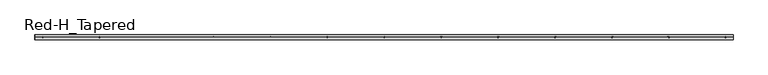
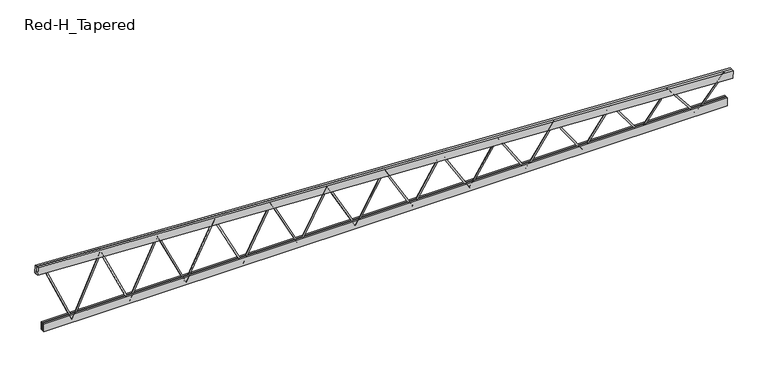
"""IFC4 building model written with IfcOpenShell, lengths in millimetres: beam geometry, Construction_Frames_RedBuilt_Openweb_Red-H_Tapered : Red-H_Tapered."""

from ifc_helpers import new_model, si_unit, point, frame, origin, origin_2d, place, context, project, spatial, polyline, circle_curve, trimmed, segment, composite_curve, outline, extrude, source, transform, mapped, element, save


def red_h_tapered_021202b6(model_context):
    return source(origin(), model_context, "Body", "SweptSolid", [
        extrude(outline(composite_curve([segment(trimmed(circle_curve(origin_2d(), 12.7), [point((0.0, 12.7))], [point((0.0, -12.7))], False, "CARTESIAN"), True, "CONTINUOUS"), segment(trimmed(circle_curve(origin_2d(), 12.7), [point((0.0, -12.7))], [point((0.0, 12.7))], False, "CARTESIAN"), True, "CONTINUOUS")], self_intersect=False)), frame((5452.665625, 0.0, -367.0101562), z_axis=(0.646986574748216, 0.0, 0.7625013915368097), x_axis=(0.0, -1.0, 0.0)), (0.0, 0.0, 1.0), 766.1625362),
        extrude(outline(composite_curve([segment(trimmed(circle_curve(origin_2d(), 12.7), [point((0.0, -12.7000001))], [point((0.0, 12.7))], False, "CARTESIAN"), True, "CONTINUOUS"), segment(trimmed(circle_curve(origin_2d(), 12.7), [point((0.0, 12.7))], [point((0.0, -12.7000001))], False, "CARTESIAN"), True, "CONTINUOUS")], self_intersect=False)), frame((5452.665625, 0.0, -367.0101562), z_axis=(-0.618861229601663, 0.0, 0.7855003364072596), x_axis=(0.0, -1.0, 0.0)), (0.0, 0.0, 1.0), 800.982274),
        extrude(outline(composite_curve([segment(trimmed(circle_curve(origin_2d(), 12.7), [point((0.0, 12.7000001))], [point((0.0, -12.7))], False, "CARTESIAN"), True, "CONTINUOUS"), segment(trimmed(circle_curve(origin_2d(), 12.7), [point((0.0, -12.7))], [point((0.0, 12.7000001))], False, "CARTESIAN"), True, "CONTINUOUS")], self_intersect=False)), frame((4461.271875, 0.0, -367.0101562), z_axis=(0.6188612296016608, 0.0, 0.7855003364072612), x_axis=(0.0, -1.0, 0.0)), (0.0, 0.0, 1.0), 800.982274),
        extrude(outline(composite_curve([segment(trimmed(circle_curve(origin_2d(), 12.7), [point((0.0, -12.7))], [point((0.0, 12.7))], False, "CARTESIAN"), True, "CONTINUOUS"), segment(trimmed(circle_curve(origin_2d(), 12.7), [point((0.0, 12.7))], [point((0.0, -12.7))], False, "CARTESIAN"), True, "CONTINUOUS")], self_intersect=False)), frame((4461.271875, 0.0, -367.0101562), z_axis=(-0.5923927653210783, 0.0, 0.8056493105534479), x_axis=(0.0, -1.0, 0.0)), (0.0, 0.0, 1.0), 836.7706428),
        extrude(outline(composite_curve([segment(trimmed(circle_curve(origin_2d(), 12.7), [point((0.0, 12.7))], [point((0.0, -12.7))], False, "CARTESIAN"), True, "CONTINUOUS"), segment(trimmed(circle_curve(origin_2d(), 12.7), [point((0.0, -12.7))], [point((0.0, 12.7))], False, "CARTESIAN"), True, "CONTINUOUS")], self_intersect=False)), frame((3469.878125, 0.0, -367.0101562), z_axis=(0.592392765321077, 0.0, 0.8056493105534488), x_axis=(0.0, -1.0, 0.0)), (0.0, 0.0, 1.0), 836.7706428),
        extrude(outline(composite_curve([segment(trimmed(circle_curve(origin_2d(), 12.7), [point((0.0, -12.7))], [point((0.0, 12.6999999))], False, "CARTESIAN"), True, "CONTINUOUS"), segment(trimmed(circle_curve(origin_2d(), 12.7), [point((0.0, 12.6999999))], [point((0.0, -12.7))], False, "CARTESIAN"), True, "CONTINUOUS")], self_intersect=False)), frame((3469.878125, 0.0, -367.0101562), z_axis=(-0.5675429419222507, 0.0, 0.8233437976169109), x_axis=(0.0, -1.0, 0.0)), (0.0, 0.0, 1.0), 873.40858),
        extrude(outline(composite_curve([segment(trimmed(circle_curve(origin_2d(), 12.7), [point((0.0, 12.7))], [point((0.0, -12.6999999))], False, "CARTESIAN"), True, "CONTINUOUS"), segment(trimmed(circle_curve(origin_2d(), 12.7), [point((0.0, -12.6999999))], [point((0.0, 12.7))], False, "CARTESIAN"), True, "CONTINUOUS")], self_intersect=False)), frame((2478.484375, 0.0, -367.0101562), z_axis=(0.5675429419222516, 0.0, 0.8233437976169103), x_axis=(0.0, -1.0, 0.0)), (0.0, 0.0, 1.0), 873.40858),
        extrude(outline(composite_curve([segment(trimmed(circle_curve(origin_2d(), 12.7), [point((0.0, -12.7000001))], [point((0.0, 12.7))], False, "CARTESIAN"), True, "CONTINUOUS"), segment(trimmed(circle_curve(origin_2d(), 12.7), [point((0.0, 12.7))], [point((0.0, -12.7000001))], False, "CARTESIAN"), True, "CONTINUOUS")], self_intersect=False)), frame((2478.484375, 0.0, -367.0101562), z_axis=(-0.5442472293507187, 0.0, 0.8389248794403861), x_axis=(0.0, -1.0, 0.0)), (0.0, 0.0, 1.0), 910.7935664),
        extrude(outline(composite_curve([segment(trimmed(circle_curve(origin_2d(), 12.7), [point((0.0, 12.7000001))], [point((0.0, -12.7))], False, "CARTESIAN"), True, "CONTINUOUS"), segment(trimmed(circle_curve(origin_2d(), 12.7), [point((0.0, -12.7))], [point((0.0, 12.7000001))], False, "CARTESIAN"), True, "CONTINUOUS")], self_intersect=False)), frame((1487.090625, 0.0, -367.0101562), z_axis=(0.5442472293507231, 0.0, 0.8389248794403832), x_axis=(0.0, -1.0, 0.0)), (0.0, 0.0, 1.0), 910.7935664),
        extrude(outline(composite_curve([segment(trimmed(circle_curve(origin_2d(), 12.7), [point((0.0, -12.7000001))], [point((0.0, 12.7))], False, "CARTESIAN"), True, "CONTINUOUS"), segment(trimmed(circle_curve(origin_2d(), 12.7), [point((0.0, 12.7))], [point((0.0, -12.7000001))], False, "CARTESIAN"), True, "CONTINUOUS")], self_intersect=False)), frame((1487.090625, 0.0, -367.0101562), z_axis=(-0.5224255765774791, 0.0, 0.8526848872459794), x_axis=(0.0, -1.0, 0.0)), (0.0, 0.0, 1.0), 948.8373028),
        extrude(outline(composite_curve([segment(trimmed(circle_curve(origin_2d(), 12.7), [point((0.0, 12.7000001))], [point((0.0, -12.7))], False, "CARTESIAN"), True, "CONTINUOUS"), segment(trimmed(circle_curve(origin_2d(), 12.7), [point((0.0, -12.7))], [point((0.0, 12.7000001))], False, "CARTESIAN"), True, "CONTINUOUS")], self_intersect=False)), frame((495.696875, 0.0, -367.0101562), z_axis=(0.5224255765774808, 0.0, 0.8526848872459784), x_axis=(0.0, -1.0, 0.0)), (0.0, 0.0, 1.0), 948.8373028),
        extrude(outline(composite_curve([segment(trimmed(circle_curve(origin_2d(), 12.7), [point((0.0, -12.7))], [point((0.0, 12.7))], False, "CARTESIAN"), True, "CONTINUOUS"), segment(trimmed(circle_curve(origin_2d(), 12.7), [point((0.0, 12.7))], [point((0.0, -12.7))], False, "CARTESIAN"), True, "CONTINUOUS")], self_intersect=False)), frame((495.696875, 0.0, -367.0101562), z_axis=(-0.5019899953354453, 0.0, 0.8648734269146668), x_axis=(0.0, -1.0, 0.0)), (0.0, 0.0, 1.0), 987.4636539),
        extrude(outline(composite_curve([segment(trimmed(circle_curve(origin_2d(), 12.7), [point((0.0, 12.7))], [point((0.0, -12.7))], False, "CARTESIAN"), True, "CONTINUOUS"), segment(trimmed(circle_curve(origin_2d(), 12.7), [point((0.0, -12.7))], [point((0.0, 12.7))], False, "CARTESIAN"), True, "CONTINUOUS")], self_intersect=False)), frame((-495.696875, 0.0, -367.0101562), z_axis=(0.5019899953354093, 0.0, 0.8648734269146878), x_axis=(0.0, -1.0, 0.0)), (0.0, 0.0, 1.0), 987.4636539),
        extrude(outline(composite_curve([segment(trimmed(circle_curve(origin_2d(), 12.7), [point((0.0, -12.7))], [point((0.0, 12.6999999))], False, "CARTESIAN"), True, "CONTINUOUS"), segment(trimmed(circle_curve(origin_2d(), 12.7), [point((0.0, 12.6999999))], [point((0.0, -12.7))], False, "CARTESIAN"), True, "CONTINUOUS")], self_intersect=False)), frame((-495.696875, 0.0, -367.0101562), z_axis=(-0.48284975973910615, 0.0, 0.8757032085814734), x_axis=(0.0, -1.0, 0.0)), (0.0, 0.0, 1.0), 1026.6068586),
        extrude(outline(composite_curve([segment(trimmed(circle_curve(origin_2d(), 12.7), [point((0.0, 12.7))], [point((0.0, -12.6999999))], False, "CARTESIAN"), True, "CONTINUOUS"), segment(trimmed(circle_curve(origin_2d(), 12.7), [point((0.0, -12.6999999))], [point((0.0, 12.7))], False, "CARTESIAN"), True, "CONTINUOUS")], self_intersect=False)), frame((-1487.090625, 0.0, -367.0101562), z_axis=(0.48284975973910677, 0.0, 0.875703208581473), x_axis=(0.0, -1.0, 0.0)), (0.0, 0.0, 1.0), 1026.6068586),
        extrude(outline(composite_curve([segment(trimmed(circle_curve(origin_2d(), 12.7), [point((0.0, -12.7))], [point((0.0, 12.7))], False, "CARTESIAN"), True, "CONTINUOUS"), segment(trimmed(circle_curve(origin_2d(), 12.7), [point((0.0, 12.7))], [point((0.0, -12.7))], False, "CARTESIAN"), True, "CONTINUOUS")], self_intersect=False)), frame((-1487.090625, 0.0, -367.0101562), z_axis=(-0.4649148648371085, 0.0, 0.885355391045592), x_axis=(0.0, -1.0, 0.0)), (0.0, 0.0, 1.0), 1066.2099935),
        extrude(outline(composite_curve([segment(trimmed(circle_curve(origin_2d(), 12.7), [point((0.0, -12.7))], [point((0.0, 12.7))], False, "CARTESIAN"), True, "CONTINUOUS"), segment(trimmed(circle_curve(origin_2d(), 12.7), [point((0.0, 12.7))], [point((0.0, -12.7))], False, "CARTESIAN"), True, "CONTINUOUS")], self_intersect=False)), frame((-2478.484375, 0.0, -367.0101562), z_axis=(0.4649148648371126, 0.0, 0.8853553910455899), x_axis=(0.0, -1.0, 0.0)), (0.0, 0.0, 1.0), 1066.2099935),
        extrude(outline(composite_curve([segment(trimmed(circle_curve(origin_2d(), 12.7), [point((0.0, 12.7))], [point((0.0, -12.7))], False, "CARTESIAN"), True, "CONTINUOUS"), segment(trimmed(circle_curve(origin_2d(), 12.7), [point((0.0, -12.7))], [point((0.0, 12.7))], False, "CARTESIAN"), True, "CONTINUOUS")], self_intersect=False)), frame((-2478.484375, 0.0, -367.0101562), z_axis=(-0.44809823878717214, 0.0, 0.8939843222315671), x_axis=(0.0, -1.0, 0.0)), (0.0, 0.0, 1.0), 1106.2236628),
        extrude(outline(composite_curve([segment(trimmed(circle_curve(origin_2d(), 12.7), [point((0.0, -12.7))], [point((0.0, 12.7))], False, "CARTESIAN"), True, "CONTINUOUS"), segment(trimmed(circle_curve(origin_2d(), 12.7), [point((0.0, 12.7))], [point((0.0, -12.7))], False, "CARTESIAN"), True, "CONTINUOUS")], self_intersect=False)), frame((-3469.878125, 0.0, -367.0101562), z_axis=(0.44809823878717164, 0.0, 0.8939843222315674), x_axis=(0.0, -1.0, 0.0)), (0.0, 0.0, 1.0), 1106.2236628),
        extrude(outline(composite_curve([segment(trimmed(circle_curve(origin_2d(), 12.7), [point((0.0, 12.6999999))], [point((0.0, -12.7))], False, "CARTESIAN"), True, "CONTINUOUS"), segment(trimmed(circle_curve(origin_2d(), 12.7), [point((0.0, -12.7))], [point((0.0, 12.6999999))], False, "CARTESIAN"), True, "CONTINUOUS")], self_intersect=False)), frame((-3469.878125, 0.0, -367.0101562), z_axis=(-0.432317078389782, 0.0, 0.9017216553529827), x_axis=(0.0, -1.0, 0.0)), (0.0, 0.0, 1.0), 1146.6048874),
        extrude(outline(composite_curve([segment(trimmed(circle_curve(origin_2d(), 12.7), [point((0.0, -12.6999999))], [point((0.0, 12.7))], False, "CARTESIAN"), True, "CONTINUOUS"), segment(trimmed(circle_curve(origin_2d(), 12.7), [point((0.0, 12.7))], [point((0.0, -12.6999999))], False, "CARTESIAN"), True, "CONTINUOUS")], self_intersect=False)), frame((-4461.271875, 0.0, -367.0101562), z_axis=(0.4323170783897885, 0.0, 0.9017216553529794), x_axis=(0.0, -1.0, 0.0)), (0.0, 0.0, 1.0), 1146.6048874),
        extrude(outline(composite_curve([segment(trimmed(circle_curve(origin_2d(), 12.7), [point((0.0, 12.7))], [point((0.0, -12.7))], False, "CARTESIAN"), True, "CONTINUOUS"), segment(trimmed(circle_curve(origin_2d(), 12.7), [point((0.0, -12.7))], [point((0.0, 12.7))], False, "CARTESIAN"), True, "CONTINUOUS")], self_intersect=False)), frame((-4461.271875, 0.0, -367.0101562), z_axis=(-0.41749357862727726, 0.0, 0.9086798731153836), x_axis=(0.0, -1.0, 0.0)), (0.0, 0.0, 1.0), 1187.3161657),
        extrude(outline(composite_curve([segment(trimmed(circle_curve(origin_2d(), 12.7), [point((0.0, -12.7))], [point((0.0, 12.7))], False, "CARTESIAN"), True, "CONTINUOUS"), segment(trimmed(circle_curve(origin_2d(), 12.7), [point((0.0, 12.7))], [point((0.0, -12.7))], False, "CARTESIAN"), True, "CONTINUOUS")], self_intersect=False)), frame((-5452.665625, 0.0, -367.0101562), z_axis=(0.41749357862727704, 0.0, 0.9086798731153837), x_axis=(0.0, -1.0, 0.0)), (0.0, 0.0, 1.0), 1187.3161657),
        extrude(outline(composite_curve([segment(trimmed(circle_curve(origin_2d(), 12.7), [point((0.0, 12.6999999))], [point((0.0, -12.7))], False, "CARTESIAN"), True, "CONTINUOUS"), segment(trimmed(circle_curve(origin_2d(), 12.7), [point((0.0, -12.7))], [point((0.0, 12.6999999))], False, "CARTESIAN"), True, "CONTINUOUS")], self_intersect=False)), frame((-5452.665625, 0.0, -367.0101562), z_axis=(-0.4035552511902556, 0.0, 0.9149552771784912), x_axis=(0.0, -1.0, 0.0)), (0.0, 0.0, 1.0), 1228.3246805),
        extrude(outline(polyline([(-5973.7625, -41.275), (-5973.7625, -3.175), (5973.7625, -3.175), (5973.7625, -41.275), (-5973.7625, -41.275)])), frame((0.0, 0.0, -386.0601562), z_axis=(0.0, 0.0, 1.0), x_axis=(1.0, 0.0, 0.0)), (0.0, 0.0, 1.0), 139.7),
        extrude(outline(polyline([(-5973.7625, 3.175), (-5973.7625, 41.275), (5973.7625, 41.275), (5973.7625, 3.175), (-5973.7625, 3.175)])), frame((0.0, 0.0, -386.0601562), z_axis=(0.0, 0.0, 1.0), x_axis=(1.0, 0.0, 0.0)), (0.0, 0.0, 1.0), 139.7),
        extrude(outline(polyline([(0.0, -38.1), (0.0, 0.0), (12166.0071587, 0.0), (12166.0071587, -38.1), (0.0, -38.1)])), frame((-6082.3624235, -3.175, 693.6153259), z_axis=(0.050106825686347715, 0.0, 0.9987438640710831), x_axis=(0.9987438640710831, 0.0, -0.050106825686347715)), (0.0, 0.0, 1.0), 139.7),
        extrude(outline(polyline([(0.0, -38.1), (0.0, 0.0), (12166.0071587, 0.0), (12166.0071587, -38.1), (0.0, -38.1)])), frame((-6082.3624235, 41.275, 693.6153259), z_axis=(0.050106825686347715, 0.0, 0.9987438640710831), x_axis=(0.9987438640710831, 0.0, -0.050106825686347715)), (0.0, 0.0, 1.0), 139.7),
    ])


if __name__ == "__main__":
    model = new_model("IFC4")
    model_context = context("Model", 3, world=origin())
    ifc_project = project(units=[si_unit("LENGTHUNIT", "METRE", prefix="MILLI")], contexts=[model_context])
    site = spatial("IfcSite", under=ifc_project)
    building = spatial("IfcBuilding", under=site)
    placement = place(None, origin())
    red_h_tapered_shape = red_h_tapered_021202b6(model_context)
    element("IfcBeam", 1, ObjectType="Construction_Frames_RedBuilt_Openweb_Red-H_Tapered : Red-H_Tapered", at=placement, inside=building, context=model_context, shape_type="MappedRepresentation", body=[
        mapped(red_h_tapered_shape, transform((0.0, 0.0, 0.0), x_axis=(1.0, 0.0, 0.0), y_axis=(0.0, 1.0, 0.0), z_axis=(0.0, 0.0, 1.0))),
    ])
    save(model, "model.ifc")

# Revit data of these elements
# Project information
#   Project Issue Date = "05/02/2019"
#   Project Status = "Project Status"
#   Client Name = "Owner"
#   Project Address = "SOMERS, WI"
#   Project Name = "OAKFIRE 2.0"
#   Project Number = "Project Number"
# Type "Construction_Frames_RedBuilt_Openweb_Red-H_Tapered : Red-H_Tapered"
#   Youtube clip = ""
#   Weight Net (Kg) = "0"
#   Webs = "Up to 2\" diameter tubular steel"
#   Uniformat II Description = ""
#   Uniformat II Code = ""
#   Uniclass 2015 Name = "Softwood trusses"
#   Uniclass 2015 Code = "Pr_20_85_90_81"
#   Uniclass 2.0 Description = "Structural Framing Systems"
#   Uniclass 2.0 Code = "SS-15-10-75"
#   Uniclass 1.4 Description = "Trusses"
#   Uniclass 1.4 Code = "L3523"
#   UNSPSC Code = "30103606"
#   Technical description = "http://www.redbuilt.com/reference/literature-and-other-resources"
#   Region South America = "None"
#   Region Oceania = "None"
#   Region North America = "US"
#   Region Middle East = "None"
#   Region Europe = "None"
#   Region Asia = "None"
#   Region Antarctica = "None"
#   Region Africa = "None"
#   QR code = "http://bimobject.com/redbuilt/product/redbuilt-0003"
#   Product url = "http://www.redbuilt.com/products/default.aspx?id=2"
#   Product group = "Wood Trusses"
#   Product family = "Construction"
#   Product data url = "https://bimobject.com/redbuilt/product/redbuilt-0003"
#   Product certification = ""
#   Product SKU = "redbuilt-0003"
#   Product Page URL = "http://www.redbuilt.com/commercial-systems/red-m-red-h-open-web-trusses"
#   Product Guid = "2c5793f2-6ffb-4665-b825-cf90c048e711"
#   Product Documentation Link = "http://www.redbuilt.com/documents/OW_Guide_2017_07_LowRes_wLinks.pdf"
#   OmniClass Description = "Wood Trusses"
#   OmniClass Code = "23-13 35 19 13 17"
#   NBS Reference Description = ""
#   NBS Reference Code = ""
#   Material secondary = "Steel"
#   Material main = "Wood"
#   Masterformat 2014 Description = "Metal-Web Wood Joists"
#   Masterformat 2014 Code = "06 17 36"
#   Manufacturer name = "RedBuilt"
#   Manufacturer country = "United States"
#   Installation instructions = "http://www.redbuilt.com/documents/Installation_Sheets_Open-Web.pdf"
#   IFC Classification = ""
#   EAN code = ""
#   Design country = "United States"
#   Product Information = "http://redbuilt.com/products/default.aspx?id=2"
#   Model = "Red-H-Tapered"
#   Manufacturer URL = "http://redbuilt.com/"
#   Manufacturer = "RedBuilt™"
#   Description = "Open Web Truss"
#   Date of publishing = "8/17/2010"
#   Contact us = "http://redbuilt.com/contact/"
#   Chords = "Double 1½\" x 5½\" MSR lumber"
#   COBIe Type Category = ""
#   Brand url = "http://www.redbuilt.com"
#   BIMobject main category code = "construction"
#   BIMobject main category = "Construction"
#   BIMobject category code = "construction-frames-trusses"
#   BIMobject category = "Frames & Trusses"
#   Web Radius = 0' - 0 1/2"
#   Web Layout Offset Start [instance default] = 0' - 5"
#   Web Layout Offset End [instance default] = 0' - 5"
#   Web Diameter = 0' - 1"
#   TotalLength [instance default] = 20' - 0"
#   Span Minimum = 4' - 0"
#   Span Maximum = 70' - 0"
#   Span Limit [instance default] = 20' - 0"
#   Nominal width = 0' - 0"
#   Nominal height = 0' - 0"
#   Inner Depth Top [instance default] = 0' - 2.76372"
#   Depth Start [instance default] = 6' - 0"
#   Top Chord Length [instance default] = 20' - 1.19701"
#   TC Extension Start Aux [instance default] = 0' - 0"
#   TC Extension End Aux [instance default] = 0' - 0"
#   T-B Chord Length Difference L [instance default] = 0' - 4"
#   T-B Chord Length Difference [instance default] = 0' - 4"
#   Height 2 [instance default] = 6' - 0"
#   Depth Minimum at Wall = 2' - 0"
#   Depth Maximum at Wall = 6' - 0"
#   Depth Lower End [instance default] = 2' - 0"
#   Depth Higher End [instance default] = 6' - 0"
#   Depth End [instance default] = 2' - 0"
#   Depth 2 [instance default] = 2' - 0"
#   Chord Width = 0' - 3 1/4"
#   Chord Thickness = 0' - 1 1/2"
#   Chord Depth = 0' - 5 1/2"
#   Offset Start [instance default] = 0' - 0"
#   TC Extension Start [instance default] = 0' - 0"
#   End Panel = 0' - 5"
#   Offset End [instance default] = 0' - 0"
#   TC Extension End [instance default] = 0' - 0"
#   Length [instance default] = 20' - 0"
#   Angle [instance default] = 5.71059°
#   Span Limit Warning [instance default] = no
#   Edition number = 1
#   Top Bearing Start [instance default] = yes
#   Top Bearing End [instance default] = yes
#   Bottom Bearing Start [instance default] = no
#   Bottom Bearing End [instance default] = no
#   8 Panels [instance default] = yes
#   16 Panels [instance default] = no
#   12 Panels [instance default] = no
#   Web Material = RedBuilt-Steel, Galvanized
#   Clip Material = RedBuilt-Steel, Galvanized
#   Chords Material = RedBuilt-MSR
#   URL = ""
#   Assembly Code = ""
# Element 1 (IfcBeam, "Construction_Frames_RedBuilt_Openweb_Red-H_Tapered : Red-H_Tapered")
#   TotalLength = 39' - 10 3/8"
#   Span Limit = 39' - 10 3/8"
#   Inner Depth Top = 0' - 2.75346"
#   Top Chord Length = 39' - 10.97666"
#   Angle = 2.87211°
#   8 Panels = no
#   12 Panels = yes
#   Materials on its faces: "RedBuilt-Steel, Galvanized", "RedBuilt-MSR"
# Materials
#   "RedBuilt-Steel, Galvanized": class "Metal", colour RGB 164 172 176, transparency 0, Manufacturer = "RedBuilt. LLC", Comments = "Openweb Metal Web", URL = "http://www.redbuilt.com/", Description = "Galvanized steel", Cost = 0
#   "RedBuilt-MSR": class "Wood", colour RGB 213 182 136, transparency 0, Manufacturer = "RedBuilt, LLC", URL = "http://www.redbuilt.com/", Cost = 0
